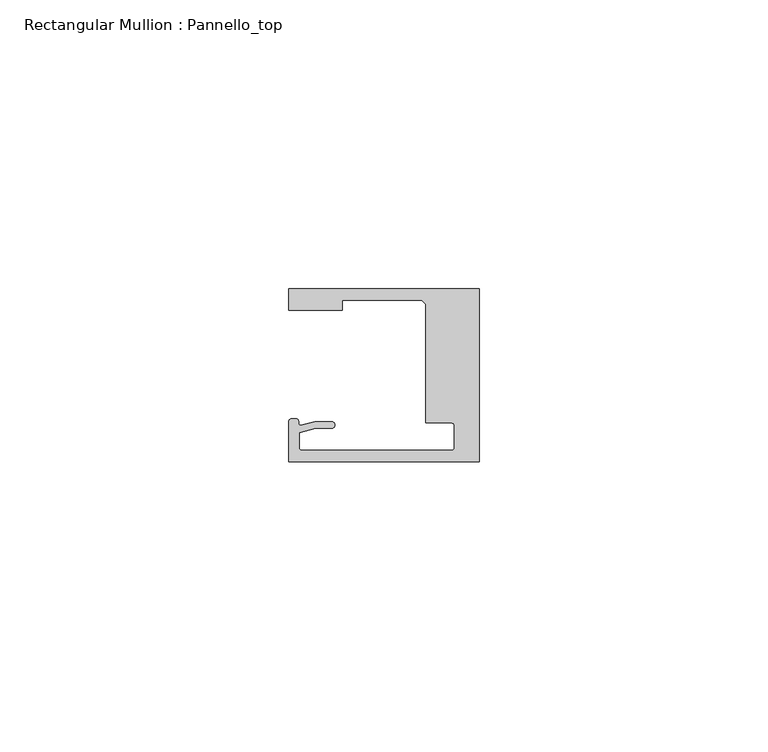
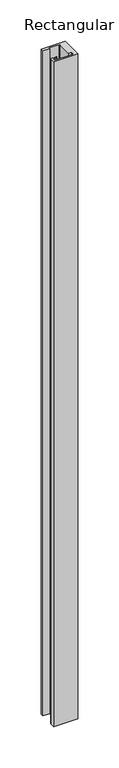
"""IFC4 building model written with IfcOpenShell, lengths in millimetres: member geometry, Rectangular Mullion : Pannello_top."""

from ifc_helpers import new_model, si_unit, frame, origin, place, context, project, spatial, polyline, circle_curve, source, transform, mapped, element, save
from ifc_brep_helpers import plane_surface, cylinder_surface, revolved_surface, extruded_surface, spline_curve, advanced_brep


def rectangular_mullion_pannello_top_b108ece7(model_context):
    return source(origin(), model_context, "Body", "AdvancedBrep", [
        advanced_brep(
        [(-33.0, 15.0, 0.0), (-33.0, 11.3000004, 0.0), (-23.700041, 11.3000004, 0.0), (-23.700041, 13.0000004, 0.0), (-10.0000103, 13.0000004, 0.0), (-9.2999726, 12.2999849, 0.0), (-9.2999726, -8.2500595, 0.0), (-4.7999726, -8.2500595, 0.0), (-4.2999726, -8.7500595, 0.0), (-4.2999726, -12.50001, 0.0), (-4.7999726, -13.00001, 0.0), (-30.69998, -13.00001, 0.0), (-31.19998, -12.50001, 0.0), (-31.19998, -9.9657591, 0.0), (-28.3419477, -9.1999523, 0.0), (-25.59998, -9.1999523, 0.0), (-25.59998, -7.9999523, 0.0), (-28.4999305, -7.9999523, 0.0), (-30.9223017, -8.6490241, 0.0), (-33.0000135, -8.0000472, 0.0), (-33.0000135, -15.0, 0.0), (0.0, -15.0, 0.0), (0.0, 15.0, 0.0), (-33.0, 15.0, -980.0), (0.0, 15.0, -980.0), (0.0, -15.0, -980.0), (-33.0000135, -15.0, -980.0), (-33.0000135, -8.0000472, -980.0), (-30.9223017, -8.6490241, -980.0), (-28.4999305, -7.9999523, -980.0), (-25.59998, -7.9999523, -980.0), (-25.59998, -9.1999523, -980.0), (-28.3419477, -9.1999523, -980.0), (-31.19998, -9.9657591, -980.0), (-31.19998, -12.50001, -980.0), (-30.69998, -13.00001, -980.0), (-4.7999726, -13.00001, -980.0), (-4.2999726, -12.50001, -980.0), (-4.2999726, -8.7500595, -980.0), (-4.7999726, -8.2500595, -980.0), (-9.2999726, -8.2500595, -980.0), (-9.2999726, 12.2999849, -980.0), (-10.0000103, 13.0000004, -980.0), (-23.700041, 13.0000004, -980.0), (-23.700041, 11.3000004, -980.0), (-33.0, 11.3000004, -980.0)],
        [
            (0, 1),
            (1, 2),
            (2, 3),
            (3, 4),
            (4, 5),
            (5, 6),
            (6, 7),
            (7, 8, circle_curve(frame((-4.7999726, -8.7500595, 0.0), z_axis=(0.0, 0.0, -1.0), x_axis=(0.0, 1.0, 0.0)), 0.5)),
            (8, 9),
            (9, 10, circle_curve(frame((-4.7999726, -12.50001, 0.0), z_axis=(0.0, 0.0, -1.0), x_axis=(1.0, 0.0, 0.0)), 0.5)),
            (10, 11),
            (11, 12, circle_curve(frame((-30.69998, -12.50001, 0.0), z_axis=(0.0, 0.0, -1.0), x_axis=(0.0, -1.0, 0.0)), 0.5)),
            (12, 13),
            (13, 14),
            (14, 15),
            (15, 16, circle_curve(frame((-25.59998, -8.5999523, 0.0), z_axis=(0.0, 0.0, 1.0), x_axis=(0.0, -1.0, 0.0)), 0.6)),
            (16, 17),
            (17, 18),
            (18, 19, spline_curve(3, [(-30.9223017, -8.6490241, 0.0), (-31.312054066, -8.717747958, 0.0), (-31.298563602, -8.366228555, 0.0), (-31.305645054, -7.690065204, 0.0), (-31.357433266, -7.563996614, 0.0), (-32.262327879, -7.456527435, 0.0), (-33.0000135, -7.457047519, 0.0), (-33.0000135, -8.0000472, 0.0)], [4, 2, 2, 4], [0.0, 0.001840817752199412, 0.004996616814974408, 0.007702013405570312])),
            (19, 20),
            (20, 21),
            (21, 22),
            (22, 0),
            (23, 24),
            (24, 25),
            (25, 26),
            (26, 27),
            (27, 28, spline_curve(3, [(-33.0000135, -8.0000472, -980.0), (-33.0000135, -7.457047519, -980.0), (-32.262327879, -7.456527435, -980.0), (-31.357433266, -7.563996614, -980.0), (-31.305645054, -7.690065204, -980.0), (-31.298563602, -8.366228555, -980.0), (-31.312054066, -8.717747958, -980.0), (-30.9223017, -8.6490241, -980.0)], [4, 2, 2, 4], [0.0, 0.0027053965905959043, 0.0058611956533709, 0.007702013405570312])),
            (28, 29),
            (29, 30),
            (30, 31, circle_curve(frame((-25.59998, -8.5999523, -980.0), z_axis=(0.0, 0.0, -1.0), x_axis=(0.0, -1.0, 0.0)), 0.6)),
            (31, 32),
            (32, 33),
            (33, 34),
            (34, 35, circle_curve(frame((-30.69998, -12.50001, -980.0), z_axis=(0.0, 0.0, 1.0), x_axis=(0.0, -1.0, 0.0)), 0.5)),
            (35, 36),
            (36, 37, circle_curve(frame((-4.7999726, -12.50001, -980.0), z_axis=(0.0, 0.0, 1.0), x_axis=(1.0, 0.0, 0.0)), 0.5)),
            (37, 38),
            (38, 39, circle_curve(frame((-4.7999726, -8.7500595, -980.0), z_axis=(0.0, 0.0, 1.0), x_axis=(0.0, 1.0, 0.0)), 0.5)),
            (39, 40),
            (40, 41),
            (41, 42),
            (42, 43),
            (43, 44),
            (44, 45),
            (45, 23),
            (0, 23),
            (45, 1),
            (44, 2),
            (43, 3),
            (42, 4),
            (41, 5),
            (40, 6),
            (39, 7),
            (38, 8),
            (37, 9),
            (36, 10),
            (35, 11),
            (34, 12),
            (33, 13),
            (32, 14),
            (31, 15),
            (30, 16),
            (29, 17),
            (28, 18),
            (27, 19),
            (26, 20),
            (25, 21),
            (24, 22),
        ],
        [
            plane_surface(frame((0.0, -36.2491502, 0.0), z_axis=(0.0, 0.0, 1.0), x_axis=(-1.0, 0.0, 0.0))),
            plane_surface(frame((0.0, -36.2491502, -980.0), z_axis=(0.0, 0.0, -1.0), x_axis=(-1.0, 0.0, 0.0))),
            plane_surface(frame((-33.0, 15.0, 0.0), z_axis=(-1.0, 0.0, 0.0), x_axis=(0.0, 0.0, -1.0))),
            plane_surface(frame((-33.0, 11.3000004, 0.0), z_axis=(0.0, -1.0, 0.0), x_axis=(0.0, 0.0, -1.0))),
            plane_surface(frame((-23.700041, 11.3000004, 0.0), z_axis=(1.0, 0.0, 0.0), x_axis=(0.0, 0.0, -1.0))),
            plane_surface(frame((-23.700041, 13.0000004, 0.0), z_axis=(0.0, -1.0, 0.0), x_axis=(0.0, 0.0, -1.0))),
            plane_surface(frame((-10.0000103, 13.0000004, 0.0), z_axis=(-0.7070955486277984, -0.7071180135668678, 0.0), x_axis=(0.0, 0.0, -1.0))),
            plane_surface(frame((-9.2999726, 12.2999849, 0.0), z_axis=(-1.0, 0.0, 0.0), x_axis=(0.0, 0.0, -1.0))),
            plane_surface(frame((-9.2999726, -8.2500595, 0.0), z_axis=(0.0, -1.0, 0.0), x_axis=(0.0, 0.0, -1.0))),
            revolved_surface(polyline([(-4.7999726, -8.2500595, -980.0), (-4.7999726, -8.2500595, 0.0)]), (-4.7999726, -8.7500595, 0.0), (0.0, 0.0, -1.0)),
            plane_surface(frame((-4.2999726, -8.7500595, 0.0), z_axis=(-1.0, 0.0, 0.0), x_axis=(0.0, 0.0, -1.0))),
            revolved_surface(polyline([(-4.2999726, -12.50001, -980.0), (-4.2999726, -12.50001, 0.0)]), (-4.7999726, -12.50001, 0.0), (0.0, 0.0, -1.0)),
            plane_surface(frame((-4.7999726, -13.00001, 0.0), z_axis=(0.0, 1.0, 0.0), x_axis=(0.0, 0.0, -1.0))),
            revolved_surface(polyline([(-30.69998, -13.00001, -980.0), (-30.69998, -13.00001, 0.0)]), (-30.69998, -12.50001, 0.0), (0.0, 0.0, -1.0)),
            plane_surface(frame((-31.19998, -12.50001, 0.0), z_axis=(1.0, 0.0, 0.0), x_axis=(0.0, 0.0, -1.0))),
            plane_surface(frame((-31.19998, -9.9657591, 0.0), z_axis=(0.25881883204288636, -0.9659258833782002, 0.0), x_axis=(0.0, 0.0, -1.0))),
            plane_surface(frame((-28.3419477, -9.1999523, 0.0), z_axis=(0.0, -1.0, 0.0), x_axis=(0.0, 0.0, -1.0))),
            cylinder_surface(frame((-25.59998, -8.5999523, 0.0), z_axis=(0.0, 0.0, 1.0), x_axis=(0.0, -1.0, 0.0)), 0.6),
            plane_surface(frame((-25.59998, -7.9999523, 0.0), z_axis=(0.0, 1.0, 0.0), x_axis=(0.0, 0.0, -1.0))),
            plane_surface(frame((-28.4999305, -7.9999523, 0.0), z_axis=(-0.25881883200192934, 0.9659258833891746, 0.0), x_axis=(0.0, 0.0, -1.0))),
            extruded_surface(spline_curve(3, [(-30.9223017, -8.6490241, -980.0), (-31.312054066, -8.717747958, -980.0), (-31.298563602, -8.366228555, -980.0), (-31.305645054, -7.690065204, -980.0), (-31.357433266, -7.563996614, -980.0), (-32.262327879, -7.456527435, -980.0), (-33.0000135, -7.457047519, -980.0), (-33.0000135, -8.0000472, -980.0)], [4, 2, 2, 4], [0.0, 0.001840817752199412, 0.004996616814974408, 0.007702013405570312]), (0.0, 0.0, 980.0), 980.0),
            plane_surface(frame((-33.0000135, -8.0000472, 0.0), z_axis=(-1.0, 0.0, 0.0), x_axis=(0.0, 0.0, -1.0))),
            plane_surface(frame((-33.0000135, -15.0, 0.0), z_axis=(0.0, -1.0, 0.0), x_axis=(0.0, 0.0, -1.0))),
            plane_surface(frame((0.0, -15.0, 0.0), z_axis=(1.0, 0.0, 0.0), x_axis=(0.0, 0.0, -1.0))),
            plane_surface(frame((0.0, 15.0, 0.0), z_axis=(0.0, 1.0, 0.0), x_axis=(0.0, 0.0, -1.0))),
        ],
        [
            (0, [[1, 2, 3, 4, 5, 6, 7, 8, 9, 10, 11, 12, 13, 14, 15, 16, 17, 18, 19, 20, 21, 22, 23]]),
            (1, [[24, 25, 26, 27, 28, 29, 30, 31, 32, 33, 34, 35, 36, 37, 38, 39, 40, 41, 42, 43, 44, 45, 46]]),
            (2, [[-1, 47, -46, 48]]),
            (3, [[-2, -48, -45, 49]]),
            (4, [[-3, -49, -44, 50]]),
            (5, [[-4, -50, -43, 51]]),
            (6, [[-5, -51, -42, 52]]),
            (7, [[-6, -52, -41, 53]]),
            (8, [[-7, -53, -40, 54]]),
            (9, [[-8, -54, -39, 55]]),
            (10, [[-9, -55, -38, 56]]),
            (11, [[-10, -56, -37, 57]]),
            (12, [[-11, -57, -36, 58]]),
            (13, [[-12, -58, -35, 59]]),
            (14, [[-13, -59, -34, 60]]),
            (15, [[-14, -60, -33, 61]]),
            (16, [[-15, -61, -32, 62]]),
            (17, [[-16, -62, -31, 63]]),
            (18, [[-17, -63, -30, 64]]),
            (19, [[-18, -64, -29, 65]]),
            (20, [[-19, -65, -28, 66]]),
            (21, [[-20, -66, -27, 67]]),
            (22, [[-21, -67, -26, 68]]),
            (23, [[-22, -68, -25, 69]]),
            (24, [[-23, -69, -24, -47]]),
        ],
    ),
    ])


if __name__ == "__main__":
    model = new_model("IFC4")
    model_context = context("Model", 3, world=origin())
    ifc_project = project(units=[si_unit("LENGTHUNIT", "METRE", prefix="MILLI")], contexts=[model_context])
    site = spatial("IfcSite", under=ifc_project)
    building = spatial("IfcBuilding", under=site)
    placement = place(None, origin())
    rectangular_mullion_pannello_top_shape = rectangular_mullion_pannello_top_b108ece7(model_context)
    element("IfcMember", 1, ObjectType="Rectangular Mullion : Pannello_top", at=placement, inside=building, context=model_context, shape_type="MappedRepresentation", body=[
        mapped(rectangular_mullion_pannello_top_shape, transform((0.0, 0.0, 0.0), x_axis=(1.0, 0.0, 0.0), y_axis=(0.0, 1.0, 0.0), z_axis=(0.0, 0.0, 1.0))),
    ])
    save(model, "model.ifc")

# Revit data of these elements
# Type "Rectangular Mullion : Pannello_top"
#   built-in parameter 1007322 = 0.0984252 (stored number, unit not read)
#   built-in parameter 1007321 = 0 (stored number, unit not read)
#   built-in parameter 1007320 = 0.0305117 (stored number, unit not read)
